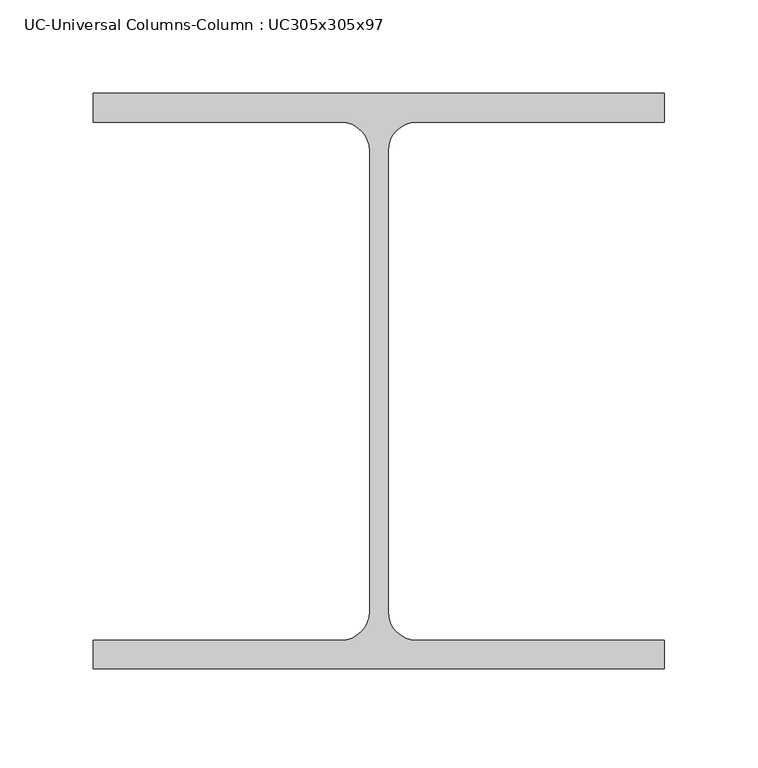
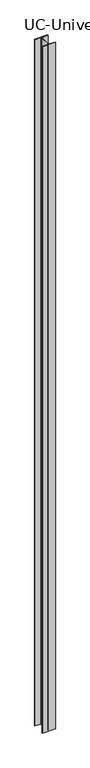
"""IFC4 building model written with IfcOpenShell, lengths in millimetres: column geometry, UC-Universal Columns-Column : UC305x305x97."""

from ifc_helpers import new_model, si_unit, point, frame, frame_2d, origin, place, context, project, spatial, polyline, circle_curve, trimmed, segment, composite_curve, outline, extrude, source, transform, mapped, element, save


def uc_universal_columns_column_uc305x305x97_02d5a26a(model_context):
    return source(origin(), model_context, "Body", "SweptSolid", [
        extrude(outline(composite_curve([segment(polyline([(152.65, 153.95), (152.65, 138.55), (20.15, 138.55)]), True, "CONTINUOUS"), segment(trimmed(circle_curve(frame_2d((20.15, 123.35)), 15.2), [point((20.15, 138.55))], [point((4.95, 123.35))], True, "CARTESIAN"), True, "CONTINUOUS"), segment(polyline([(4.95, 123.35), (4.95, -123.35)]), True, "CONTINUOUS"), segment(trimmed(circle_curve(frame_2d((20.15, -123.35)), 15.2), [point((4.95, -123.35))], [point((20.15, -138.55))], True, "CARTESIAN"), True, "CONTINUOUS"), segment(polyline([(20.15, -138.55), (152.65, -138.55), (152.65, -153.95), (-152.65, -153.95), (-152.65, -138.55), (-20.15, -138.55)]), True, "CONTINUOUS"), segment(trimmed(circle_curve(frame_2d((-20.15, -123.35)), 15.2), [point((-20.15, -138.55))], [point((-4.95, -123.35))], True, "CARTESIAN"), True, "CONTINUOUS"), segment(polyline([(-4.95, -123.35), (-4.95, 123.35)]), True, "CONTINUOUS"), segment(trimmed(circle_curve(frame_2d((-20.15, 123.35)), 15.2), [point((-4.95, 123.35))], [point((-20.15, 138.55))], True, "CARTESIAN"), True, "CONTINUOUS"), segment(polyline([(-20.15, 138.55), (-152.65, 138.55), (-152.65, 153.95), (152.65, 153.95)]), True, "CONTINUOUS")], self_intersect=False)), frame((0.0, 0.0, -4550.0), z_axis=(0.0, 0.0, 1.0), x_axis=(1.0, 0.0, 0.0)), (0.0, 0.0, 1.0), 16989.0),
    ])


if __name__ == "__main__":
    model = new_model("IFC4")
    model_context = context("Model", 3, world=origin())
    ifc_project = project(units=[si_unit("LENGTHUNIT", "METRE", prefix="MILLI")], contexts=[model_context])
    site = spatial("IfcSite", under=ifc_project)
    building = spatial("IfcBuilding", under=site)
    placement = place(None, origin())
    uc_universal_columns_column_uc305x305x97_shape = uc_universal_columns_column_uc305x305x97_02d5a26a(model_context)
    element("IfcColumn", 1, ObjectType="UC-Universal Columns-Column : UC305x305x97", at=placement, inside=building, context=model_context, shape_type="MappedRepresentation", body=[
        mapped(uc_universal_columns_column_uc305x305x97_shape, transform((0.0, 0.0, 0.0), x_axis=(1.0, 0.0, 0.0), y_axis=(0.0, 1.0, 0.0), z_axis=(0.0, 0.0, 1.0))),
    ])
    save(model, "model.ifc")

# Revit data of these elements
# Type "UC-Universal Columns-Column : UC305x305x97"
#   Section Name Key = "UC305x305x97"
#   Cost = 2
#   Width = 30.53 cm
#   Web Thickness = 0.99 cm
#   Web Fillet = 1.52 cm
#   Warping Constant = 1560000.0 cm⁶
#   Torsional Moment of Inertia = 91.20 cm⁴
#   Section Area = 123.0 cm²
#   Plastic Modulus weak axis = 726.0 cm³
#   Plastic Modulus strong axis = 1592.0 cm³
#   Nominal Weight = 96.8996 kgf/m
#   Moment of Inertia weak axis = 7308.00 cm⁴
#   Moment of Inertia strong axis = 22249.00 cm⁴
#   Height = 30.79 cm
#   Flange Thickness = 1.54 cm
#   Elastic Modulus weak axis = 479.0 cm³
#   Elastic Modulus strong axis = 1445.0 cm³
#   Centroid Vertical = 15.395 cm
#   Centroid Horizontal = 15.265 cm
#   Bolt Spacing = 14.0 cm
#   Structural Material [instance default] = Metal - Steel 43-275
#   Type Comments = ""
#   Assembly Code = ""
# Element 1 (IfcColumn, "UC-Universal Columns-Column : UC305x305x97")
#   Materials on its faces: "Metal - Steel 43-275"
# Materials
#   "Metal - Steel 43-275": class "Metal", colour RGB 247 247 247, transparency 0, Cost = 0
